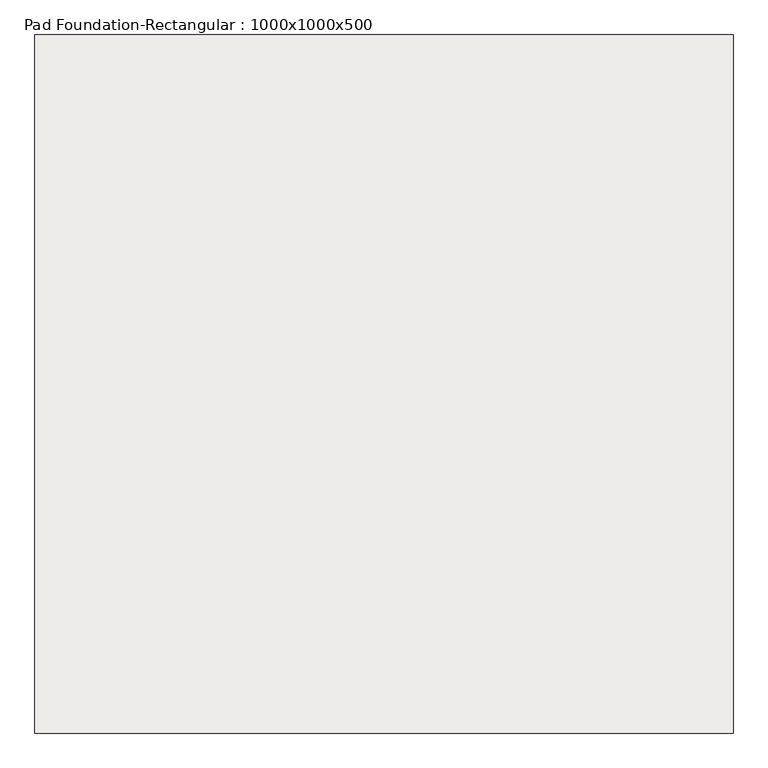
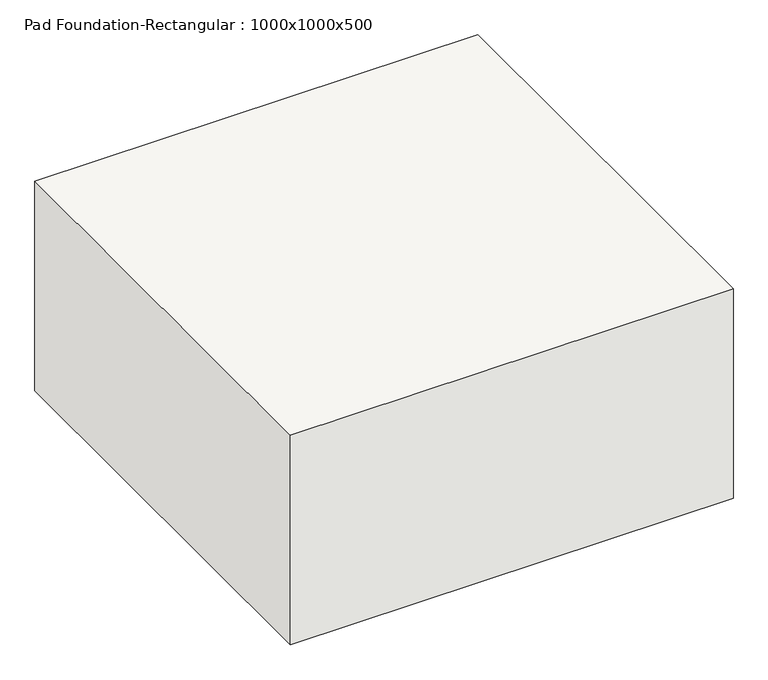
"""IFC4 building model written with IfcOpenShell, lengths in millimetres: slab geometry, Pad Foundation-Rectangular : 1000x1000x500."""

from ifc_helpers import new_model, si_unit, frame, origin, place, context, project, spatial, polyline, outline, extrude, source, transform, mapped, element, save


def pad_foundation_rectangular_1000x1000x500_ed6229e9(model_context):
    return source(origin(), model_context, "Body", "SweptSolid", [
        extrude(outline(polyline([(500.0, 500.0), (500.0, -500.0), (-500.0, -500.0), (-500.0, 500.0), (500.0, 500.0)])), frame((0.0, 0.0, -500.0), z_axis=(0.0, 0.0, 1.0), x_axis=(1.0, 0.0, 0.0)), (0.0, 0.0, 1.0), 500.0),
    ])


if __name__ == "__main__":
    model = new_model("IFC4")
    model_context = context("Model", 3, world=origin())
    ifc_project = project(units=[si_unit("LENGTHUNIT", "METRE", prefix="MILLI")], contexts=[model_context])
    site = spatial("IfcSite", under=ifc_project)
    building = spatial("IfcBuilding", under=site)
    placement = place(None, origin())
    pad_foundation_rectangular_1000x1000x500_shape = pad_foundation_rectangular_1000x1000x500_ed6229e9(model_context)
    element("IfcSlab", 1, ObjectType="Pad Foundation-Rectangular : 1000x1000x500", at=placement, inside=building, context=model_context, shape_type="MappedRepresentation", body=[
        mapped(pad_foundation_rectangular_1000x1000x500_shape, transform((0.0, 0.0, 0.0), x_axis=(1.0, 0.0, 0.0), y_axis=(0.0, 1.0, 0.0), z_axis=(0.0, 0.0, 1.0))),
    ])
    save(model, "model.ifc")

# Revit data of these elements
# Type "Pad Foundation-Rectangular : 1000x1000x500"
#   Reinforcement Specs [instance default] = ""
#   Pad Type = "P1"
#   Mesh [instance default] = ""
#   Concrete Grade [instance default] = ""
#   Volume = 0.50 m³
#   Pad Width = 1000 mm
#   Pad Length = 1000 mm
#   Pad Depth = 500 mm
#   Structural Material [instance default] = Concrete - Cast-in-Place Concrete
# Element 1 (IfcSlab, "Pad Foundation-Rectangular : 1000x1000x500")
#   Materials on its faces: "Concrete - Cast-in-Place Concrete"
# Materials
#   "Concrete - Cast-in-Place Concrete": class "Concrete", colour RGB 192 192 192, transparency 0
